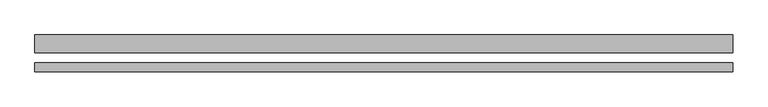
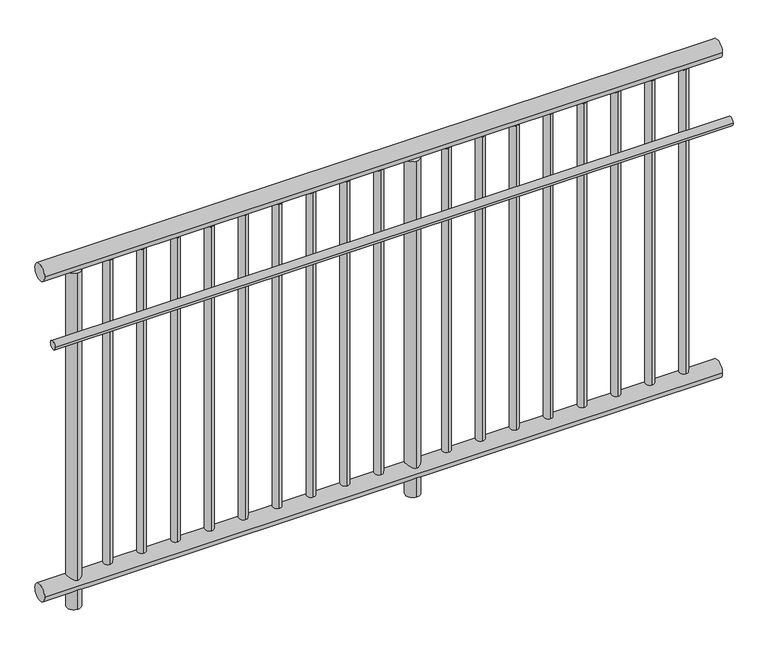
"""IFC4 building model written with IfcOpenShell, lengths in millimetres: railing geometry."""

from ifc_helpers import new_model, si_unit, point, frame, frame_2d, origin, origin_with_axes, place, context, project, spatial, circle_curve, trimmed, segment, composite_curve, outline, extrude, source, transform, mapped, element, save


def railing_a54e72fa(model_context):
    return source(origin(), model_context, "Body", "SweptSolid", [
        extrude(outline(composite_curve([segment(trimmed(circle_curve(frame_2d((30348.1400611, 1074.6)), 25.4), [point((30373.5400611, 1074.6))], [point((30322.7400611, 1074.6))], False, "CARTESIAN"), True, "CONTINUOUS"), segment(trimmed(circle_curve(frame_2d((30348.1400611, 1074.6)), 25.4), [point((30322.7400611, 1074.6))], [point((30373.5400611, 1074.6))], False, "CARTESIAN"), True, "CONTINUOUS")], self_intersect=False)), frame((9666.6129185, 0.0, 0.0), z_axis=(1.0, 0.0, 0.0), x_axis=(0.0, 1.0, 0.0)), (0.0, 0.0, 1.0), 2000.0),
        extrude(outline(composite_curve([segment(trimmed(circle_curve(frame_2d((30281.1400611, 887.3)), 12.7), [point((30293.8400611, 887.3))], [point((30268.4400611, 887.3))], False, "CARTESIAN"), True, "CONTINUOUS"), segment(trimmed(circle_curve(frame_2d((30281.1400611, 887.3)), 12.7), [point((30268.4400611, 887.3))], [point((30293.8400611, 887.3))], False, "CARTESIAN"), True, "CONTINUOUS")], self_intersect=False)), frame((9666.6129185, 0.0, 0.0), z_axis=(1.0, 0.0, 0.0), x_axis=(0.0, 1.0, 0.0)), (0.0, 0.0, 1.0), 2000.0),
        extrude(outline(composite_curve([segment(trimmed(circle_curve(frame_2d((30348.1400611, 74.6)), 25.4), [point((30373.5400611, 74.6))], [point((30322.7400611, 74.6))], False, "CARTESIAN"), True, "CONTINUOUS"), segment(trimmed(circle_curve(frame_2d((30348.1400611, 74.6)), 25.4), [point((30322.7400611, 74.6))], [point((30373.5400611, 74.6))], False, "CARTESIAN"), True, "CONTINUOUS")], self_intersect=False)), frame((9666.6129185, 0.0, 0.0), z_axis=(1.0, 0.0, 0.0), x_axis=(0.0, 1.0, 0.0)), (0.0, 0.0, 1.0), 2000.0),
        extrude(outline(composite_curve([segment(trimmed(circle_curve(frame_2d((11566.6129185, 30348.1400611)), 12.5), [point((11566.6129185, 30360.6400611))], [point((11566.6129185, 30335.6400611))], False, "CARTESIAN"), True, "CONTINUOUS"), segment(trimmed(circle_curve(frame_2d((11566.6129185, 30348.1400611)), 12.5), [point((11566.6129185, 30335.6400611))], [point((11566.6129185, 30360.6400611))], False, "CARTESIAN"), True, "CONTINUOUS")], self_intersect=False)), frame((0.0, 0.0, 100.0), z_axis=(0.0, 0.0, 1.0), x_axis=(1.0, 0.0, 0.0)), (0.0, 0.0, 1.0), 949.2),
        extrude(outline(composite_curve([segment(trimmed(circle_curve(frame_2d((11466.6129185, 30348.1400611)), 12.5), [point((11466.6129185, 30360.6400611))], [point((11466.6129185, 30335.6400611))], False, "CARTESIAN"), True, "CONTINUOUS"), segment(trimmed(circle_curve(frame_2d((11466.6129185, 30348.1400611)), 12.5), [point((11466.6129185, 30335.6400611))], [point((11466.6129185, 30360.6400611))], False, "CARTESIAN"), True, "CONTINUOUS")], self_intersect=False)), frame((0.0, 0.0, 100.0), z_axis=(0.0, 0.0, 1.0), x_axis=(1.0, 0.0, 0.0)), (0.0, 0.0, 1.0), 949.2),
        extrude(outline(composite_curve([segment(trimmed(circle_curve(frame_2d((11366.6129185, 30348.1400611)), 12.5), [point((11366.6129185, 30360.6400611))], [point((11366.6129185, 30335.6400611))], False, "CARTESIAN"), True, "CONTINUOUS"), segment(trimmed(circle_curve(frame_2d((11366.6129185, 30348.1400611)), 12.5), [point((11366.6129185, 30335.6400611))], [point((11366.6129185, 30360.6400611))], False, "CARTESIAN"), True, "CONTINUOUS")], self_intersect=False)), frame((0.0, 0.0, 100.0), z_axis=(0.0, 0.0, 1.0), x_axis=(1.0, 0.0, 0.0)), (0.0, 0.0, 1.0), 949.2),
        extrude(outline(composite_curve([segment(trimmed(circle_curve(frame_2d((11266.6129185, 30348.1400611)), 12.5), [point((11266.6129185, 30360.6400611))], [point((11266.6129185, 30335.6400611))], False, "CARTESIAN"), True, "CONTINUOUS"), segment(trimmed(circle_curve(frame_2d((11266.6129185, 30348.1400611)), 12.5), [point((11266.6129185, 30335.6400611))], [point((11266.6129185, 30360.6400611))], False, "CARTESIAN"), True, "CONTINUOUS")], self_intersect=False)), frame((0.0, 0.0, 100.0), z_axis=(0.0, 0.0, 1.0), x_axis=(1.0, 0.0, 0.0)), (0.0, 0.0, 1.0), 949.2),
        extrude(outline(composite_curve([segment(trimmed(circle_curve(frame_2d((11166.6129185, 30348.1400611)), 12.5), [point((11166.6129185, 30360.6400611))], [point((11166.6129185, 30335.6400611))], False, "CARTESIAN"), True, "CONTINUOUS"), segment(trimmed(circle_curve(frame_2d((11166.6129185, 30348.1400611)), 12.5), [point((11166.6129185, 30335.6400611))], [point((11166.6129185, 30360.6400611))], False, "CARTESIAN"), True, "CONTINUOUS")], self_intersect=False)), frame((0.0, 0.0, 100.0), z_axis=(0.0, 0.0, 1.0), x_axis=(1.0, 0.0, 0.0)), (0.0, 0.0, 1.0), 949.2),
        extrude(outline(composite_curve([segment(trimmed(circle_curve(frame_2d((11066.6129185, 30348.1400611)), 12.5), [point((11066.6129185, 30360.6400611))], [point((11066.6129185, 30335.6400611))], False, "CARTESIAN"), True, "CONTINUOUS"), segment(trimmed(circle_curve(frame_2d((11066.6129185, 30348.1400611)), 12.5), [point((11066.6129185, 30335.6400611))], [point((11066.6129185, 30360.6400611))], False, "CARTESIAN"), True, "CONTINUOUS")], self_intersect=False)), frame((0.0, 0.0, 100.0), z_axis=(0.0, 0.0, 1.0), x_axis=(1.0, 0.0, 0.0)), (0.0, 0.0, 1.0), 949.2),
        extrude(outline(composite_curve([segment(trimmed(circle_curve(frame_2d((10966.6129185, 30348.1400611)), 12.5), [point((10966.6129185, 30360.6400611))], [point((10966.6129185, 30335.6400611))], False, "CARTESIAN"), True, "CONTINUOUS"), segment(trimmed(circle_curve(frame_2d((10966.6129185, 30348.1400611)), 12.5), [point((10966.6129185, 30335.6400611))], [point((10966.6129185, 30360.6400611))], False, "CARTESIAN"), True, "CONTINUOUS")], self_intersect=False)), frame((0.0, 0.0, 100.0), z_axis=(0.0, 0.0, 1.0), x_axis=(1.0, 0.0, 0.0)), (0.0, 0.0, 1.0), 949.2),
        extrude(outline(composite_curve([segment(trimmed(circle_curve(frame_2d((10866.6129185, 30348.1400611)), 12.5), [point((10866.6129185, 30360.6400611))], [point((10866.6129185, 30335.6400611))], False, "CARTESIAN"), True, "CONTINUOUS"), segment(trimmed(circle_curve(frame_2d((10866.6129185, 30348.1400611)), 12.5), [point((10866.6129185, 30335.6400611))], [point((10866.6129185, 30360.6400611))], False, "CARTESIAN"), True, "CONTINUOUS")], self_intersect=False)), frame((0.0, 0.0, 100.0), z_axis=(0.0, 0.0, 1.0), x_axis=(1.0, 0.0, 0.0)), (0.0, 0.0, 1.0), 949.2),
        extrude(outline(composite_curve([segment(trimmed(circle_curve(frame_2d((10766.6129185, 30348.1400611)), 21.0), [point((10766.6129185, 30369.1400611))], [point((10766.6129185, 30327.1400611))], False, "CARTESIAN"), True, "CONTINUOUS"), segment(trimmed(circle_curve(frame_2d((10766.6129185, 30348.1400611)), 21.0), [point((10766.6129185, 30327.1400611))], [point((10766.6129185, 30369.1400611))], False, "CARTESIAN"), True, "CONTINUOUS")], self_intersect=False)), origin_with_axes(), (0.0, 0.0, 1.0), 1049.2),
        extrude(outline(composite_curve([segment(trimmed(circle_curve(frame_2d((10666.6129185, 30348.1400611)), 12.5), [point((10666.6129185, 30360.6400611))], [point((10666.6129185, 30335.6400611))], False, "CARTESIAN"), True, "CONTINUOUS"), segment(trimmed(circle_curve(frame_2d((10666.6129185, 30348.1400611)), 12.5), [point((10666.6129185, 30335.6400611))], [point((10666.6129185, 30360.6400611))], False, "CARTESIAN"), True, "CONTINUOUS")], self_intersect=False)), frame((0.0, 0.0, 100.0), z_axis=(0.0, 0.0, 1.0), x_axis=(1.0, 0.0, 0.0)), (0.0, 0.0, 1.0), 949.2),
        extrude(outline(composite_curve([segment(trimmed(circle_curve(frame_2d((10566.6129185, 30348.1400611)), 12.5), [point((10566.6129185, 30360.6400611))], [point((10566.6129185, 30335.6400611))], False, "CARTESIAN"), True, "CONTINUOUS"), segment(trimmed(circle_curve(frame_2d((10566.6129185, 30348.1400611)), 12.5), [point((10566.6129185, 30335.6400611))], [point((10566.6129185, 30360.6400611))], False, "CARTESIAN"), True, "CONTINUOUS")], self_intersect=False)), frame((0.0, 0.0, 100.0), z_axis=(0.0, 0.0, 1.0), x_axis=(1.0, 0.0, 0.0)), (0.0, 0.0, 1.0), 949.2),
        extrude(outline(composite_curve([segment(trimmed(circle_curve(frame_2d((10466.6129185, 30348.1400611)), 12.5), [point((10466.6129185, 30360.6400611))], [point((10466.6129185, 30335.6400611))], False, "CARTESIAN"), True, "CONTINUOUS"), segment(trimmed(circle_curve(frame_2d((10466.6129185, 30348.1400611)), 12.5), [point((10466.6129185, 30335.6400611))], [point((10466.6129185, 30360.6400611))], False, "CARTESIAN"), True, "CONTINUOUS")], self_intersect=False)), frame((0.0, 0.0, 100.0), z_axis=(0.0, 0.0, 1.0), x_axis=(1.0, 0.0, 0.0)), (0.0, 0.0, 1.0), 949.2),
        extrude(outline(composite_curve([segment(trimmed(circle_curve(frame_2d((10366.6129185, 30348.1400611)), 12.5), [point((10366.6129185, 30360.6400611))], [point((10366.6129185, 30335.6400611))], False, "CARTESIAN"), True, "CONTINUOUS"), segment(trimmed(circle_curve(frame_2d((10366.6129185, 30348.1400611)), 12.5), [point((10366.6129185, 30335.6400611))], [point((10366.6129185, 30360.6400611))], False, "CARTESIAN"), True, "CONTINUOUS")], self_intersect=False)), frame((0.0, 0.0, 100.0), z_axis=(0.0, 0.0, 1.0), x_axis=(1.0, 0.0, 0.0)), (0.0, 0.0, 1.0), 949.2),
        extrude(outline(composite_curve([segment(trimmed(circle_curve(frame_2d((10266.6129185, 30348.1400611)), 12.5), [point((10266.6129185, 30360.6400611))], [point((10266.6129185, 30335.6400611))], False, "CARTESIAN"), True, "CONTINUOUS"), segment(trimmed(circle_curve(frame_2d((10266.6129185, 30348.1400611)), 12.5), [point((10266.6129185, 30335.6400611))], [point((10266.6129185, 30360.6400611))], False, "CARTESIAN"), True, "CONTINUOUS")], self_intersect=False)), frame((0.0, 0.0, 100.0), z_axis=(0.0, 0.0, 1.0), x_axis=(1.0, 0.0, 0.0)), (0.0, 0.0, 1.0), 949.2),
        extrude(outline(composite_curve([segment(trimmed(circle_curve(frame_2d((10166.6129185, 30348.1400611)), 12.5), [point((10166.6129185, 30360.6400611))], [point((10166.6129185, 30335.6400611))], False, "CARTESIAN"), True, "CONTINUOUS"), segment(trimmed(circle_curve(frame_2d((10166.6129185, 30348.1400611)), 12.5), [point((10166.6129185, 30335.6400611))], [point((10166.6129185, 30360.6400611))], False, "CARTESIAN"), True, "CONTINUOUS")], self_intersect=False)), frame((0.0, 0.0, 100.0), z_axis=(0.0, 0.0, 1.0), x_axis=(1.0, 0.0, 0.0)), (0.0, 0.0, 1.0), 949.2),
        extrude(outline(composite_curve([segment(trimmed(circle_curve(frame_2d((10066.6129185, 30348.1400611)), 12.5), [point((10066.6129185, 30360.6400611))], [point((10066.6129185, 30335.6400611))], False, "CARTESIAN"), True, "CONTINUOUS"), segment(trimmed(circle_curve(frame_2d((10066.6129185, 30348.1400611)), 12.5), [point((10066.6129185, 30335.6400611))], [point((10066.6129185, 30360.6400611))], False, "CARTESIAN"), True, "CONTINUOUS")], self_intersect=False)), frame((0.0, 0.0, 100.0), z_axis=(0.0, 0.0, 1.0), x_axis=(1.0, 0.0, 0.0)), (0.0, 0.0, 1.0), 949.2),
        extrude(outline(composite_curve([segment(trimmed(circle_curve(frame_2d((9966.6129185, 30348.1400611)), 12.5), [point((9966.6129185, 30360.6400611))], [point((9966.6129185, 30335.6400611))], False, "CARTESIAN"), True, "CONTINUOUS"), segment(trimmed(circle_curve(frame_2d((9966.6129185, 30348.1400611)), 12.5), [point((9966.6129185, 30335.6400611))], [point((9966.6129185, 30360.6400611))], False, "CARTESIAN"), True, "CONTINUOUS")], self_intersect=False)), frame((0.0, 0.0, 100.0), z_axis=(0.0, 0.0, 1.0), x_axis=(1.0, 0.0, 0.0)), (0.0, 0.0, 1.0), 949.2),
        extrude(outline(composite_curve([segment(trimmed(circle_curve(frame_2d((9866.6129185, 30348.1400611)), 12.5), [point((9866.6129185, 30360.6400611))], [point((9866.6129185, 30335.6400611))], False, "CARTESIAN"), True, "CONTINUOUS"), segment(trimmed(circle_curve(frame_2d((9866.6129185, 30348.1400611)), 12.5), [point((9866.6129185, 30335.6400611))], [point((9866.6129185, 30360.6400611))], False, "CARTESIAN"), True, "CONTINUOUS")], self_intersect=False)), frame((0.0, 0.0, 100.0), z_axis=(0.0, 0.0, 1.0), x_axis=(1.0, 0.0, 0.0)), (0.0, 0.0, 1.0), 949.2),
        extrude(outline(composite_curve([segment(trimmed(circle_curve(frame_2d((9766.6129185, 30348.1400611)), 21.0), [point((9766.6129185, 30369.1400611))], [point((9766.6129185, 30327.1400611))], False, "CARTESIAN"), True, "CONTINUOUS"), segment(trimmed(circle_curve(frame_2d((9766.6129185, 30348.1400611)), 21.0), [point((9766.6129185, 30327.1400611))], [point((9766.6129185, 30369.1400611))], False, "CARTESIAN"), True, "CONTINUOUS")], self_intersect=False)), origin_with_axes(), (0.0, 0.0, 1.0), 1049.2),
    ])


if __name__ == "__main__":
    model = new_model("IFC4")
    model_context = context("Model", 3, world=origin())
    ifc_project = project(units=[si_unit("LENGTHUNIT", "METRE", prefix="MILLI")], contexts=[model_context])
    site = spatial("IfcSite", under=ifc_project)
    building = spatial("IfcBuilding", under=site)
    placement = place(None, origin())
    railing_shape = railing_a54e72fa(model_context)
    element("IfcRailing", 1, at=placement, inside=building, context=model_context, shape_type="MappedRepresentation", body=[
        mapped(railing_shape, transform((0.0, 0.0, 0.0), x_axis=(1.0, 0.0, 0.0), y_axis=(0.0, 1.0, 0.0), z_axis=(0.0, 0.0, 1.0))),
    ])
    save(model, "model.ifc")

# Revit data of these elements
# Element 1 (IfcRailing)
#   Materials on its faces: "Ferro - Pintura Esmalte"
# Materials
#   "Ferro - Pintura Esmalte": class "Pintura", colour RGB 255 255 255, transparency 0, Cost = 0
